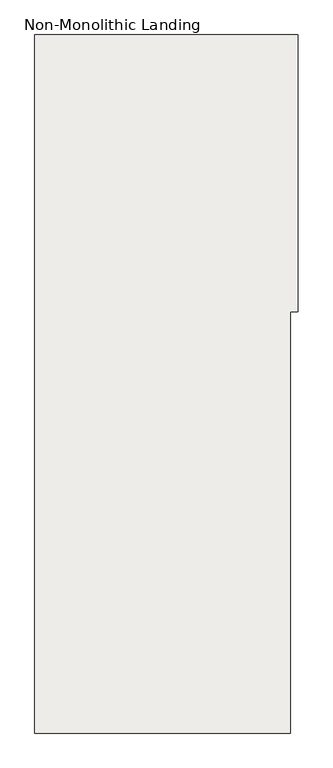
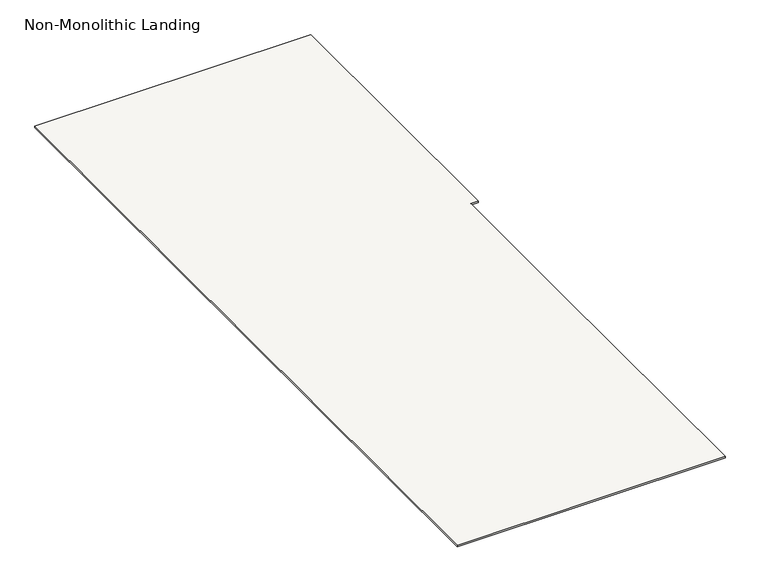
"""IFC4 building model written with IfcOpenShell, lengths in millimetres: slab geometry, Non-Monolithic Landing."""

from ifc_helpers import new_model, si_unit, origin, place, context, project, spatial, faceted_brep, source, transform, mapped, element, save


def non_monolithic_landing_e09a6105(model_context):
    return source(origin(), model_context, "Body", "Brep", [
        faceted_brep([(-16318.9400908, 12030.4345331, 30588.2352941), (-16318.0900908, 12030.4345331, 30582.2352941), (-16318.0900908, 13220.4345331, 30582.2352941), (-16318.9400908, 13220.4345331, 30588.2352941), (-16350.0, 11395.4345331, 30588.2352941), (-16350.0, 12030.4345331, 30588.2352941), (-16350.0, 13220.4345331, 30588.2352941), (-17450.0, 13220.4345331, 30588.2352941), (-17450.0, 10220.4345331, 30588.2352941), (-16350.0, 10220.4345331, 30588.2352941), (-16350.0, 12030.4345331, 30582.2352941), (-16350.0, 11395.4345331, 30582.2352941), (-16350.85, 11395.4345331, 30582.2352941), (-16350.85, 10220.4345331, 30582.2352941), (-17450.0, 10220.4345331, 30582.2352941), (-17450.0, 13220.4345331, 30582.2352941), (-16350.0, 13220.4345331, 30582.2352941)], [[[0, 1, 2, 3]], [[4, 5, 0, 3, 6, 7, 8, 9]], [[10, 11, 12, 13, 14, 15, 16, 2, 1]], [[5, 4, 11, 10]], [[0, 5, 10, 1]], [[6, 3, 2, 16]], [[7, 6, 16, 15]], [[8, 7, 15, 14]], [[9, 8, 14, 13]], [[4, 12, 11]], [[12, 4, 9, 13]]]),
    ])


if __name__ == "__main__":
    model = new_model("IFC4")
    model_context = context("Model", 3, world=origin())
    ifc_project = project(units=[si_unit("LENGTHUNIT", "METRE", prefix="MILLI")], contexts=[model_context])
    site = spatial("IfcSite", under=ifc_project)
    building = spatial("IfcBuilding", under=site)
    placement = place(None, origin())
    non_monolithic_landing_shape = non_monolithic_landing_e09a6105(model_context)
    element("IfcSlab", 1, ObjectType="Non-Monolithic Landing", at=placement, inside=building, context=model_context, shape_type="MappedRepresentation", body=[
        mapped(non_monolithic_landing_shape, transform((0.0, 0.0, 0.0), x_axis=(1.0, 0.0, 0.0), y_axis=(0.0, 1.0, 0.0), z_axis=(0.0, 0.0, 1.0))),
    ])
    save(model, "model.ifc")

# Revit data of these elements
# Element 1 (IfcSlab, "Non-Monolithic Landing")
#   Materials on its faces: "Steel, Paint Finish, Dark Gray"
# Materials
#   "Steel, Paint Finish, Dark Gray": class "Metal", colour RGB 89 89 89, transparency 0, Description = "Steel, paint finish, dark gray, glossy", Cost = 0
